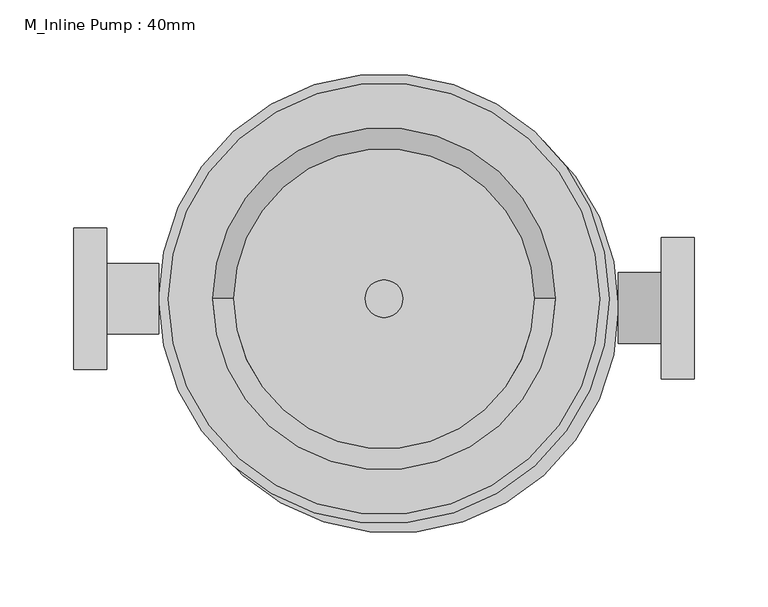
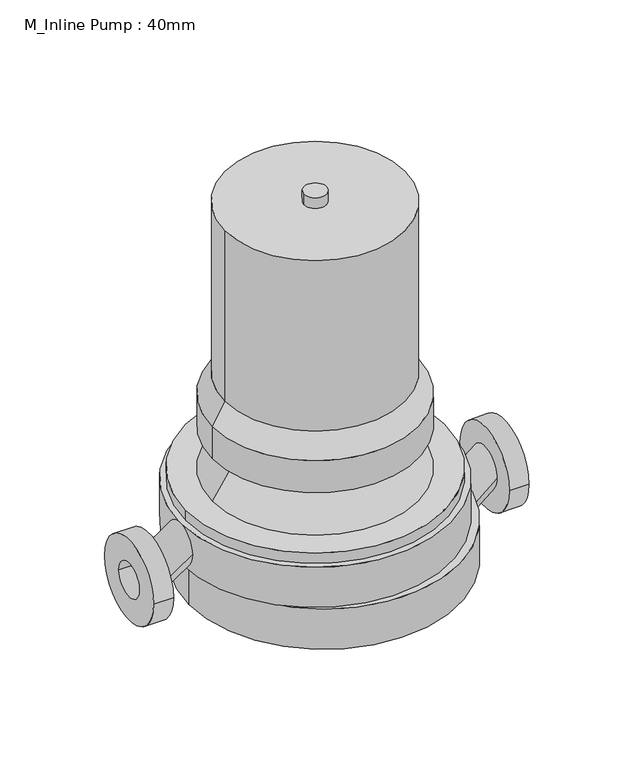
"""IFC4 building model written with IfcOpenShell, lengths in millimetres: proxy geometry, M_Inline Pump : 40mm."""

from ifc_helpers import new_model, si_unit, point, frame, frame_2d, origin, origin_with_axes, origin_2d, place, context, project, spatial, polyline, circle_curve, trimmed, segment, composite_curve, outline, extrude, source, transform, mapped, element, save
from ifc_brep_helpers import plane_surface, revolved_surface, extruded_surface, advanced_brep


def m_inline_pump_40mm_89dae234(model_context):
    return source(origin(), model_context, "Body", "SolidModel", [
        advanced_brep(
        [(158.75, -30.35, 43.0698437), (158.75, 17.65, 43.0698437), (187.7, -30.35, 67.0698438), (187.7, 17.65, 67.0698438)],
        [
            (0, 1, circle_curve(frame((158.75, -6.35, 43.0698437), z_axis=(-1.0, 0.0, 0.0), x_axis=(0.0, 1.0, 0.0)), 24.0)),
            (1, 0, circle_curve(frame((158.75, -6.35, 43.0698437), z_axis=(-1.0, 0.0, 0.0), x_axis=(0.0, 1.0, 0.0)), 24.0)),
            (2, 3, circle_curve(frame((187.7, -6.35, 67.0698438), z_axis=(1.0, 0.0, 0.0), x_axis=(0.0, 1.0, 0.0)), 24.0)),
            (3, 2, circle_curve(frame((187.7, -6.35, 67.0698438), z_axis=(1.0, 0.0, 0.0), x_axis=(0.0, 1.0, 0.0)), 24.0)),
            (3, 1),
            (0, 2),
        ],
        [
            plane_surface(frame((158.75, -6.35, 43.0698437), z_axis=(-1.0, 0.0, 0.0), x_axis=(0.0, 0.0, -1.0))),
            plane_surface(frame((187.7, -6.35, 67.0698438), z_axis=(1.0, 0.0, 0.0), x_axis=(0.0, 0.0, -1.0))),
            extruded_surface(trimmed(circle_curve(frame((187.7, -6.35, 67.0698438), z_axis=(-1.0, 0.0, 0.0), x_axis=(0.0, 1.0, 0.0)), 24.0), [point((187.7, -30.35, 67.0698438))], [point((187.7, 17.65, 67.0698438))], True, "CARTESIAN"), (-28.94999999999999, 0.0, -24.0000001), 37.604554309285454),
            extruded_surface(trimmed(circle_curve(frame((187.7, -6.35, 67.0698438), z_axis=(-1.0, 0.0, 0.0), x_axis=(0.0, 1.0, 0.0)), 24.0), [point((187.7, 17.65, 67.0698438))], [point((187.7, -30.35, 67.0698438))], True, "CARTESIAN"), (-28.94999999999999, 0.0, -24.0000001), 37.604554309285454),
        ],
        [
            (0, [[1, 2]]),
            (1, [[3, 4]]),
            (2, [[-4, 5, -1, 6]]),
            (3, [[-3, -6, -2, -5]]),
        ],
    ),
        extrude(outline(composite_curve([segment(trimmed(circle_curve(frame_2d((-6.35, 67.0698438)), 48.0), [point((-54.35, 67.0698438))], [point((41.65, 67.0698438))], False, "CARTESIAN"), True, "CONTINUOUS"), segment(trimmed(circle_curve(frame_2d((-6.35, 67.0698438)), 48.0), [point((41.65, 67.0698438))], [point((-54.35, 67.0698438))], False, "CARTESIAN"), True, "CONTINUOUS")], self_intersect=False), holes=[composite_curve([segment(trimmed(circle_curve(frame_2d((-6.35, 67.0698438)), 20.0), [point((-26.35, 67.0698438))], [point((13.65, 67.0698438))], True, "CARTESIAN"), True, "CONTINUOUS"), segment(trimmed(circle_curve(frame_2d((-6.35, 67.0698438)), 20.0), [point((13.65, 67.0698438))], [point((-26.35, 67.0698438))], True, "CARTESIAN"), True, "CONTINUOUS")], self_intersect=False)]), frame((187.7, 0.0, 0.0), z_axis=(1.0, 0.0, 0.0), x_axis=(0.0, 1.0, 0.0)), (0.0, 0.0, 1.0), 22.3),
        advanced_brep(
        [(-152.4, -24.0, 91.0698437), (-152.4, 24.0, 91.0698437), (-187.7, -24.0, 67.0698437), (-187.7, 24.0, 67.0698437)],
        [
            (0, 1, circle_curve(frame((-152.4, 0.0, 91.0698437), z_axis=(1.0, 0.0, 0.0), x_axis=(0.0, 1.0, 0.0)), 24.0)),
            (1, 0, circle_curve(frame((-152.4, 0.0, 91.0698437), z_axis=(1.0, 0.0, 0.0), x_axis=(0.0, 1.0, 0.0)), 24.0)),
            (2, 3, circle_curve(frame((-187.7, 0.0, 67.0698437), z_axis=(-1.0, 0.0, 0.0), x_axis=(0.0, 1.0, 0.0)), 24.0)),
            (3, 2, circle_curve(frame((-187.7, 0.0, 67.0698437), z_axis=(-1.0, 0.0, 0.0), x_axis=(0.0, 1.0, 0.0)), 24.0)),
            (3, 1),
            (0, 2),
        ],
        [
            plane_surface(frame((-152.4, 0.0, 91.0698437), z_axis=(1.0, 0.0, 0.0), x_axis=(0.0, 0.0, -1.0))),
            plane_surface(frame((-187.7, 0.0, 67.0698437), z_axis=(-1.0, 0.0, 0.0), x_axis=(0.0, 0.0, -1.0))),
            extruded_surface(trimmed(circle_curve(frame((-187.7, 0.0, 67.0698437), z_axis=(1.0, 0.0, 0.0), x_axis=(0.0, 1.0, 0.0)), 24.0), [point((-187.7, -24.0, 67.0698437))], [point((-187.7, 24.0, 67.0698437))], True, "CARTESIAN"), (35.29999999999998, 0.0, 24.0), 42.68594616498501),
            extruded_surface(trimmed(circle_curve(frame((-187.7, 0.0, 67.0698437), z_axis=(1.0, 0.0, 0.0), x_axis=(0.0, 1.0, 0.0)), 24.0), [point((-187.7, 24.0, 67.0698437))], [point((-187.7, -24.0, 67.0698437))], True, "CARTESIAN"), (35.29999999999998, 0.0, 24.0), 42.68594616498501),
        ],
        [
            (0, [[1, 2]]),
            (1, [[3, 4]]),
            (2, [[-4, 5, -1, 6]]),
            (3, [[-3, -6, -2, -5]]),
        ],
    ),
        extrude(outline(composite_curve([segment(trimmed(circle_curve(frame_2d((0.0, 67.0698437)), 48.0), [point((-48.0, 67.0698437))], [point((48.0, 67.0698437))], False, "CARTESIAN"), True, "CONTINUOUS"), segment(trimmed(circle_curve(frame_2d((0.0, 67.0698437)), 48.0), [point((48.0, 67.0698437))], [point((-48.0, 67.0698437))], False, "CARTESIAN"), True, "CONTINUOUS")], self_intersect=False), holes=[composite_curve([segment(trimmed(circle_curve(frame_2d((0.0, 67.0698437)), 20.0), [point((-20.0, 67.0698437))], [point((20.0, 67.0698437))], True, "CARTESIAN"), True, "CONTINUOUS"), segment(trimmed(circle_curve(frame_2d((0.0, 67.0698437)), 20.0), [point((20.0, 67.0698437))], [point((-20.0, 67.0698437))], True, "CARTESIAN"), True, "CONTINUOUS")], self_intersect=False)]), frame((-210.0, 0.0, 0.0), z_axis=(1.0, 0.0, 0.0), x_axis=(0.0, 1.0, 0.0)), (0.0, 0.0, 1.0), 22.3),
        extrude(outline(composite_curve([segment(trimmed(circle_curve(origin_2d(), 12.7), [point((-12.7, 0.0))], [point((12.7, 0.0))], False, "CARTESIAN"), True, "CONTINUOUS"), segment(trimmed(circle_curve(origin_2d(), 12.7), [point((12.7, 0.0))], [point((-12.7, 0.0))], False, "CARTESIAN"), True, "CONTINUOUS")], self_intersect=False)), frame((0.0, 0.0, 445.2698437), z_axis=(0.0, 0.0, 1.0), x_axis=(1.0, 0.0, 0.0)), (0.0, 0.0, 1.0), 12.7),
        extrude(outline(composite_curve([segment(trimmed(circle_curve(origin_2d(), 152.4), [point((-152.4, 0.0))], [point((152.4, 0.0))], False, "CARTESIAN"), True, "CONTINUOUS"), segment(trimmed(circle_curve(origin_2d(), 152.4), [point((152.4, 0.0))], [point((-152.4, 0.0))], False, "CARTESIAN"), True, "CONTINUOUS")], self_intersect=False)), frame((0.0, 0.0, 67.0698437), z_axis=(0.0, 0.0, 1.0), x_axis=(1.0, 0.0, 0.0)), (0.0, 0.0, 1.0), 48.0),
        extrude(outline(composite_curve([segment(trimmed(circle_curve(frame_2d((6.35, -6.35)), 152.4), [point((-146.05, -6.35))], [point((158.75, -6.35))], False, "CARTESIAN"), True, "CONTINUOUS"), segment(trimmed(circle_curve(frame_2d((6.35, -6.35)), 152.4), [point((158.75, -6.35))], [point((-146.05, -6.35))], False, "CARTESIAN"), True, "CONTINUOUS")], self_intersect=False)), frame((0.0, 0.0, 19.0698437), z_axis=(0.0, 0.0, 1.0), x_axis=(1.0, 0.0, 0.0)), (0.0, 0.0, 1.0), 48.0),
        extrude(outline(composite_curve([segment(trimmed(circle_curve(origin_2d(), 38.1), [point((-38.1, 0.0))], [point((38.1, 0.0))], False, "CARTESIAN"), True, "CONTINUOUS"), segment(trimmed(circle_curve(origin_2d(), 38.1), [point((38.1, 0.0))], [point((-38.1, 0.0))], False, "CARTESIAN"), True, "CONTINUOUS")], self_intersect=False)), frame((0.0, 0.0, 6.35), z_axis=(0.0, 0.0, 1.0), x_axis=(1.0, 0.0, 0.0)), (0.0, 0.0, 1.0), 12.7198437),
        extrude(outline(composite_curve([segment(trimmed(circle_curve(origin_2d(), 12.7), [point((-12.7, 0.0))], [point((12.7, 0.0))], False, "CARTESIAN"), True, "CONTINUOUS"), segment(trimmed(circle_curve(origin_2d(), 12.7), [point((12.7, 0.0))], [point((-12.7, 0.0))], False, "CARTESIAN"), True, "CONTINUOUS")], self_intersect=False)), origin_with_axes(), (0.0, 0.0, 1.0), 6.35),
        extrude(outline(composite_curve([segment(trimmed(circle_curve(origin_2d(), 101.6), [point((-101.6, 0.0))], [point((101.6, 0.0))], False, "CARTESIAN"), True, "CONTINUOUS"), segment(trimmed(circle_curve(origin_2d(), 101.6), [point((101.6, 0.0))], [point((-101.6, 0.0))], False, "CARTESIAN"), True, "CONTINUOUS")], self_intersect=False)), frame((0.0, 0.0, 242.0698437), z_axis=(0.0, 0.0, 1.0), x_axis=(1.0, 0.0, 0.0)), (0.0, 0.0, 1.0), 203.2),
        advanced_brep(
        [(-101.6, 0.0, 242.0698437), (101.6, 0.0, 242.0698437), (-115.8875, 0.0, 216.6698437), (115.8875, 0.0, 216.6698437)],
        [
            (0, 1, circle_curve(frame((0.0, 0.0, 242.0698437), z_axis=(0.0, 0.0, 1.0), x_axis=(-1.0, 0.0, 0.0)), 101.6)),
            (1, 0, circle_curve(frame((0.0, 0.0, 242.0698437), z_axis=(0.0, 0.0, 1.0), x_axis=(1.0, 0.0, 0.0)), 101.6)),
            (2, 3, circle_curve(frame((0.0, 0.0, 216.6698437), z_axis=(0.0, 0.0, -1.0), x_axis=(1.0, 0.0, 0.0)), 115.8875)),
            (3, 2, circle_curve(frame((0.0, 0.0, 216.6698437), z_axis=(0.0, 0.0, -1.0), x_axis=(-1.0, 0.0, 0.0)), 115.8875)),
            (3, 1),
            (0, 2),
        ],
        [
            plane_surface(frame((0.0, 0.0, 242.0698437), z_axis=(0.0, 0.0, 1.0), x_axis=(0.0, -1.0, 0.0))),
            plane_surface(frame((0.0, 0.0, 216.6698437), z_axis=(0.0, 0.0, -1.0), x_axis=(0.0, -1.0, 0.0))),
            revolved_surface(polyline([(-101.60000000539384, 0.0, 242.0698437), (-115.8875, 0.0, 216.6698437)]), (0.0, 0.0, 422.692066), (0.0, 0.0, -1.0)),
            revolved_surface(polyline([(101.60000000539384, 0.0, 242.0698437), (115.8875, 0.0, 216.6698437)]), (0.0, 0.0, 422.692066), (0.0, 0.0, -1.0)),
        ],
        [
            (0, [[1, 2]]),
            (1, [[3, 4]]),
            (2, [[-4, 5, -1, 6]]),
            (3, [[-3, -6, -2, -5]]),
        ],
    ),
        extrude(outline(composite_curve([segment(trimmed(circle_curve(origin_2d(), 115.8875), [point((-115.8875, 0.0))], [point((115.8875, 0.0))], False, "CARTESIAN"), True, "CONTINUOUS"), segment(trimmed(circle_curve(origin_2d(), 115.8875), [point((115.8875, 0.0))], [point((-115.8875, 0.0))], False, "CARTESIAN"), True, "CONTINUOUS")], self_intersect=False)), frame((0.0, 0.0, 178.5698437), z_axis=(0.0, 0.0, 1.0), x_axis=(1.0, 0.0, 0.0)), (0.0, 0.0, 1.0), 38.1),
        advanced_brep(
        [(-82.55, 0.0, 178.5698437), (82.55, 0.0, 178.5698437), (-115.8875, 0.0, 127.7698437), (115.8875, 0.0, 127.7698437)],
        [
            (0, 1, circle_curve(frame((0.0, 0.0, 178.5698437), z_axis=(0.0, 0.0, 1.0), x_axis=(-1.0, 0.0, 0.0)), 82.55)),
            (1, 0, circle_curve(frame((0.0, 0.0, 178.5698437), z_axis=(0.0, 0.0, 1.0), x_axis=(1.0, 0.0, 0.0)), 82.55)),
            (2, 3, circle_curve(frame((0.0, 0.0, 127.7698437), z_axis=(0.0, 0.0, -1.0), x_axis=(1.0, 0.0, 0.0)), 115.8875)),
            (3, 2, circle_curve(frame((0.0, 0.0, 127.7698437), z_axis=(0.0, 0.0, -1.0), x_axis=(-1.0, 0.0, 0.0)), 115.8875)),
            (3, 1),
            (0, 2),
        ],
        [
            plane_surface(frame((0.0, 0.0, 178.5698437), z_axis=(0.0, 0.0, 1.0), x_axis=(0.0, -1.0, 0.0))),
            plane_surface(frame((0.0, 0.0, 127.7698437), z_axis=(0.0, 0.0, -1.0), x_axis=(0.0, -1.0, 0.0))),
            revolved_surface(polyline([(-82.55000000179793, 0.0, 178.56984370000004), (-115.8875, 0.0, 127.7698437)]), (0.0, 0.0, 304.3603199), (0.0, 0.0, -1.0)),
            revolved_surface(polyline([(82.55000000179793, 0.0, 178.56984370000004), (115.8875, 0.0, 127.7698437)]), (0.0, 0.0, 304.3603199), (0.0, 0.0, -1.0)),
        ],
        [
            (0, [[1, 2]]),
            (1, [[3, 4]]),
            (2, [[-4, 5, -1, 6]]),
            (3, [[-3, -6, -2, -5]]),
        ],
    ),
        extrude(outline(composite_curve([segment(trimmed(circle_curve(origin_2d(), 146.05), [point((-146.05, 0.0))], [point((146.05, 0.0))], False, "CARTESIAN"), True, "CONTINUOUS"), segment(trimmed(circle_curve(origin_2d(), 146.05), [point((146.05, 0.0))], [point((-146.05, 0.0))], False, "CARTESIAN"), True, "CONTINUOUS")], self_intersect=False)), frame((0.0, 0.0, 115.0698437), z_axis=(0.0, 0.0, 1.0), x_axis=(1.0, 0.0, 0.0)), (0.0, 0.0, 1.0), 12.7),
    ])


if __name__ == "__main__":
    model = new_model("IFC4")
    model_context = context("Model", 3, world=origin())
    ifc_project = project(units=[si_unit("LENGTHUNIT", "METRE", prefix="MILLI")], contexts=[model_context])
    site = spatial("IfcSite", under=ifc_project)
    building = spatial("IfcBuilding", under=site)
    placement = place(None, origin())
    m_inline_pump_40mm_shape = m_inline_pump_40mm_89dae234(model_context)
    element("IfcBuildingElementProxy", 1, Name="M_Inline Pump : 40mm", ObjectType="M_Inline Pump : 40mm", at=placement, inside=building, context=model_context, shape_type="MappedRepresentation", body=[
        mapped(m_inline_pump_40mm_shape, transform((0.0, 0.0, 0.0), x_axis=(1.0, 0.0, 0.0), y_axis=(0.0, 1.0, 0.0), z_axis=(0.0, 0.0, 1.0))),
    ])
    save(model, "model.ifc")

# Revit data of these elements
# Type "M_Inline Pump : 40mm"
#   Model = "74574"
#   Manufacturer = "Grundfoss"
#   Description = "Pump"
#   COBie.Type.CreatedBy = "design@eagle.com"
#   COBie.Type.CreatedOn = "2016-09-13T05:47:35"
#   COBie.Type.Name = "Mechanical Equipment_M_Inline Pump_40mm"
#   COBie.Type.Category = "23-60 30 21 : Pumps"
#   COBie.Type.Description = "Pump"
#   COBie.Type.Manufacturer = "Grundfoss"
#   COBie.Type.ModelNumber = "74574"
#   Pump Speed = "1750"
#   COBie.Type.ReplacementCost = 0
#   Voltage = 230 V
#   Suction Radius = 20 mm
#   Suction Outside Radius = 24 mm
#   Suction Outside Diameter = 48 mm
#   Suction Nominal Diameter = 40 mm
#   Suction Flange Outside Radius = 48 mm
#   Suction Flange Outside Diameter = 96 mm
#   Suction Flange Length = 22.3 mm
#   Length = 420 mm
#   Height = 48 mm
#   Half Length = 210 mm
#   Discharge Radius = 20 mm
#   Discharge Outside Radius = 24 mm
#   Discharge Outside Diameter = 48 mm
#   Discharge Nominal Diameter = 40 mm
#   Discharge Flange Outside Radius = 48 mm
#   Discharge Flange Outside Diameter = 96 mm
#   Discharge Flange Length = 22.3 mm
#   Apparent Load = 2000 VA
#   COBie.Type = yes
#   Number of Poles = 2
#   Pump Material = none
#   Load Classification = Appliance - Dwelling Unit
